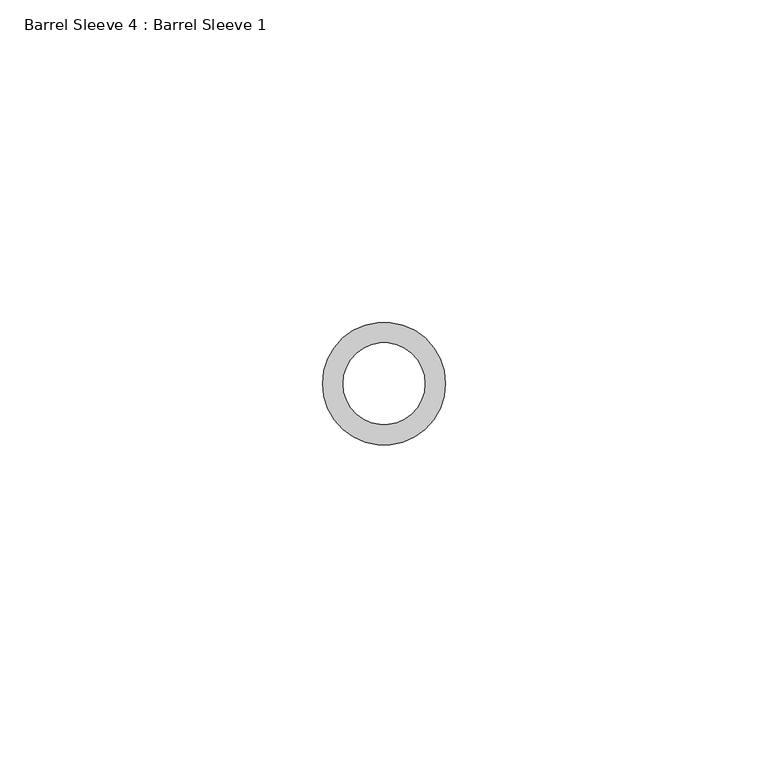
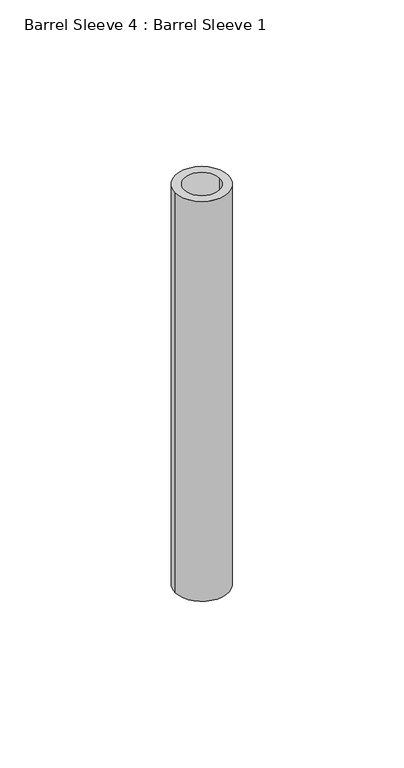
"""IFC4 building model written with IfcOpenShell, lengths in millimetres: proxy geometry, Barrel Sleeve 4 : Barrel Sleeve 1."""

from ifc_helpers import new_model, si_unit, point, frame, frame_2d, origin, place, context, project, spatial, circle_curve, trimmed, segment, composite_curve, outline, extrude, source, transform, mapped, element, save


def barrel_sleeve_4_barrel_sleeve_1_23cef5c5(model_context):
    return source(origin(), model_context, "Body", "SweptSolid", [
        extrude(outline(composite_curve([segment(trimmed(circle_curve(frame_2d((587309.5435739, -535163.4663841)), 9.525), [point((587300.0185739, -535163.4663841))], [point((587319.068574, -535163.4663841))], False, "CARTESIAN"), True, "CONTINUOUS"), segment(trimmed(circle_curve(frame_2d((587309.5435739, -535163.4663841)), 9.525), [point((587319.068574, -535163.4663841))], [point((587300.0185739, -535163.4663841))], False, "CARTESIAN"), True, "CONTINUOUS")], self_intersect=False), holes=[composite_curve([segment(trimmed(circle_curve(frame_2d((587309.5435739, -535163.4663841)), 6.35), [point((587303.1935739, -535163.4663841))], [point((587315.893574, -535163.4663841))], True, "CARTESIAN"), True, "CONTINUOUS"), segment(trimmed(circle_curve(frame_2d((587309.5435739, -535163.4663841)), 6.35), [point((587315.893574, -535163.4663841))], [point((587303.1935739, -535163.4663841))], True, "CARTESIAN"), True, "CONTINUOUS")], self_intersect=False)]), frame((0.0, 0.0, -152.4), z_axis=(0.0, 0.0, 1.0), x_axis=(1.0, 0.0, 0.0)), (0.0, 0.0, 1.0), 152.4),
    ])


if __name__ == "__main__":
    model = new_model("IFC4")
    model_context = context("Model", 3, world=origin())
    ifc_project = project(units=[si_unit("LENGTHUNIT", "METRE", prefix="MILLI")], contexts=[model_context])
    site = spatial("IfcSite", under=ifc_project)
    building = spatial("IfcBuilding", under=site)
    placement = place(None, origin())
    barrel_sleeve_4_barrel_sleeve_1_shape = barrel_sleeve_4_barrel_sleeve_1_23cef5c5(model_context)
    element("IfcBuildingElementProxy", 1, Name="Barrel Sleeve 4 : Barrel Sleeve 1", ObjectType="Barrel Sleeve 4 : Barrel Sleeve 1", at=placement, inside=building, context=model_context, shape_type="MappedRepresentation", body=[
        mapped(barrel_sleeve_4_barrel_sleeve_1_shape, transform((0.0, 0.0, 0.0), x_axis=(1.0, 0.0, 0.0), y_axis=(0.0, 1.0, 0.0), z_axis=(0.0, 0.0, 1.0))),
    ])
    save(model, "model.ifc")

# Revit data of these elements
# Element 1 (IfcBuildingElementProxy, "Barrel Sleeve 4 : Barrel Sleeve 1")
#   Materials on its faces: "5/8\" ID STEEL SLEEVE"
# Materials
#   "5/8\" ID STEEL SLEEVE": class "Metal", colour RGB 189 187 185, transparency 0, Description = "Carbon steel", Cost = 0
